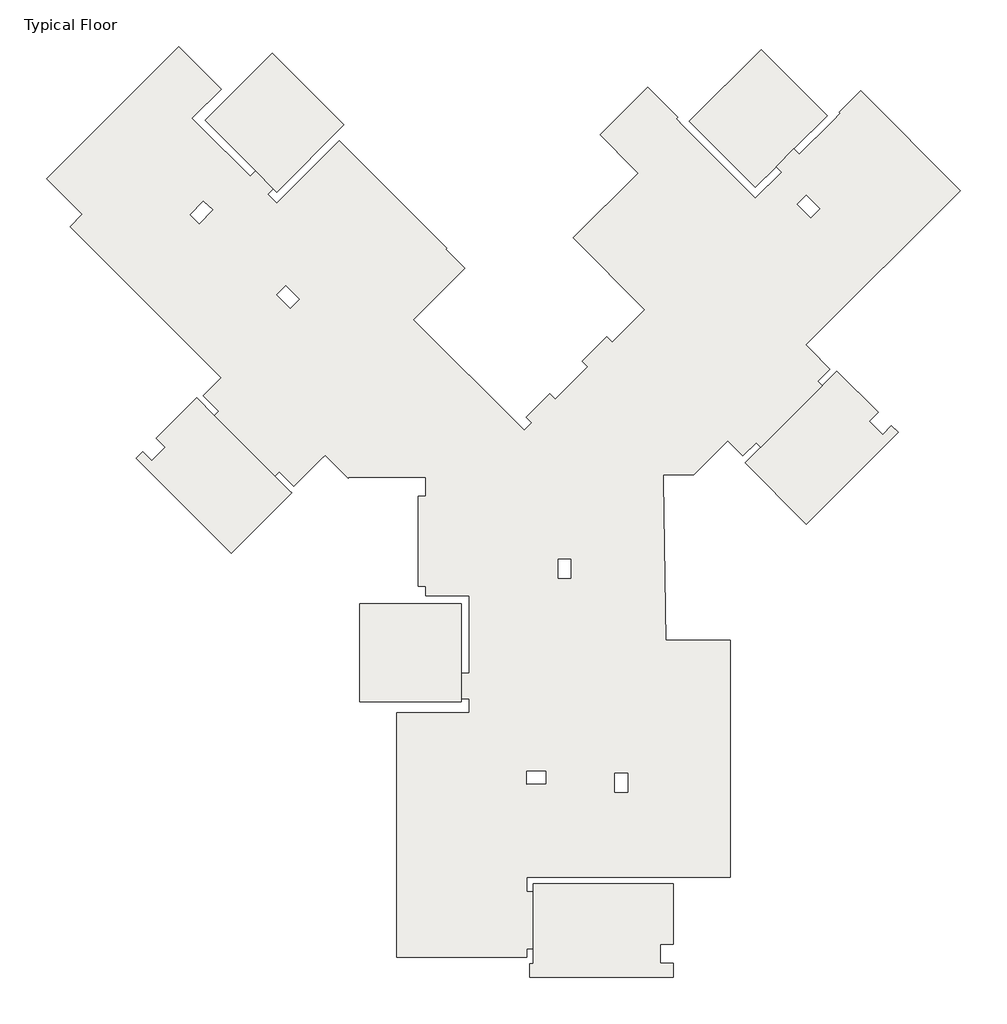
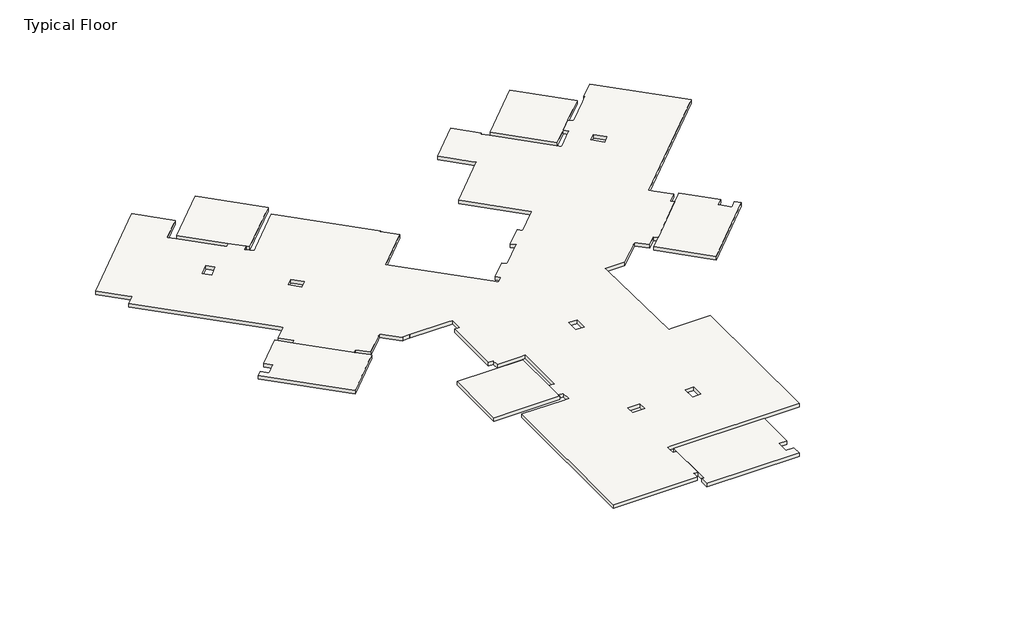
# One storey: 7 slabs.
"""IFC4 building model written with IfcOpenShell, lengths in millimetres."""

from ifc_helpers import new_model, si_unit, origin, place, context, project, spatial, faceted_brep, element, save

model = new_model("IFC4")

# Units and contexts
model_context = context("Model", 3, world=origin())
ifc_project = project(units=[si_unit("LENGTHUNIT", "METRE", prefix="MILLI")], contexts=[model_context])

# Site, building, storey
site = spatial("IfcSite", under=ifc_project)
building = spatial("IfcBuilding", under=site)
storey = spatial("IfcBuildingStorey", under=building, Name="Typical Floor", Elevation=3000.0)

# Slabs
placement = place(None, origin())
element("IfcSlab", 1, ObjectType="18", at=placement, inside=storey, context=model_context, shape_type="Brep", body=[
    faceted_brep([(-7856.4284934, -710.7469277, 2820.0), (-10855.8752998, 2291.0608544, 2820.0), (-10643.7250884, 2503.0442058, 2820.0), (-10362.7349591, 2221.337265, 2820.0), (-9937.9307713, 2645.0605261, 2820.0), (-10219.2939768, 2927.1414948, 2820.0), (-8946.5252944, 4198.9091219, 2820.0), (-8385.3549973, 3637.7388248, 2820.0), (-6476.6083787, 1728.9922062, 2820.0), (-6010.9986053, 1263.3824328, 2820.0), (-5945.8975357, 1198.2813632, 2820.0), (-10855.8752998, 2291.0608544, 3000.0), (-7856.4284934, -710.7469277, 3000.0), (-5945.8975357, 1198.2813632, 3000.0), (-6010.9986053, 1263.3824328, 3000.0), (-6476.6083787, 1728.9922062, 3000.0), (-8385.3549973, 3637.7388248, 3000.0), (-8946.5252944, 4198.9091219, 3000.0), (-10219.2939768, 2927.1414948, 3000.0), (-9937.9307713, 2645.0605261, 3000.0), (-10362.7349591, 2221.337265, 3000.0), (-10643.7250884, 2503.0442058, 3000.0)], [[[0, 1, 2, 3, 4, 5, 6, 7, 8, 9, 10]], [[11, 12, 13, 14, 15, 16, 17, 18, 19, 20, 21]], [[1, 0, 12, 11]], [[1, 11, 21, 2]], [[17, 6, 5, 18]], [[6, 17, 16, 15, 14, 13, 10, 9, 8, 7]], [[0, 10, 13, 12]], [[3, 20, 19, 4]], [[20, 3, 2, 21]], [[4, 19, 18, 5]]]),
])
element("IfcSlab", 2, ObjectType="18", at=placement, inside=storey, context=model_context, shape_type="Brep", body=[
    faceted_brep([(1689.535885, -11158.0646121, 2820.0), (6112.9804297, -11158.0646121, 2820.0), (6112.9804297, -13069.1556852, 2820.0), (5712.9804297, -13069.1556852, 2820.0), (5712.9804297, -13669.1556852, 2820.0), (6112.9804297, -13669.1556852, 2820.0), (6112.9804297, -14118.5695716, 2820.0), (1589.2653711, -14118.5695716, 2820.0), (1589.2653711, -13687.1899503, 2820.0), (1689.535885, -13687.1899503, 2820.0), (1689.535885, -13208.1998691, 2820.0), (1689.535885, -11409.1015824, 2820.0), (6112.9804297, -11158.0646121, 3000.0), (1689.535885, -11158.0646121, 3000.0), (1689.535885, -11409.1015824, 3000.0), (1689.535885, -13208.1998691, 3000.0), (1689.535885, -13687.1899503, 3000.0), (1589.2653711, -13687.1899503, 3000.0), (1589.2653711, -14118.5695716, 3000.0), (6112.9804297, -14118.5695716, 3000.0), (6112.9804297, -13669.1556852, 3000.0), (5712.9804297, -13669.1556852, 3000.0), (5712.9804297, -13069.1556852, 3000.0), (6112.9804297, -13069.1556852, 3000.0)], [[[0, 1, 2, 3, 4, 5, 6, 7, 8, 9, 10, 11]], [[12, 13, 14, 15, 16, 17, 18, 19, 20, 21, 22, 23]], [[1, 0, 13, 12]], [[1, 12, 23, 2]], [[19, 6, 5, 20]], [[7, 6, 19, 18]], [[8, 7, 18, 17]], [[9, 8, 17, 16]], [[9, 16, 15, 14, 13, 0, 11, 10]], [[4, 21, 20, 5]], [[21, 4, 3, 22]], [[22, 3, 2, 23]]]),
])
element("IfcSlab", 3, ObjectType="18", at=placement, inside=storey, context=model_context, shape_type="Brep", body=[
    faceted_brep([(13230.1629629, 3112.966169, 2820.0), (10331.02516, 213.8283661, 2820.0), (8393.4317005, 2151.4218256, 2820.0), (8888.8145144, 2646.8046394, 2820.0), (10826.9573797, 4584.9475048, 2820.0), (11210.8737714, 4968.8638964, 2820.0), (11292.5695034, 5050.5596284, 2820.0), (12593.7668598, 3749.362272, 2820.0), (12310.9241473, 3466.5195596, 2820.0), (12735.188216, 3042.2554908, 2820.0), (13018.0309285, 3325.0982033, 2820.0), (10331.02516, 213.8283661, 3000.0), (13230.1629629, 3112.966169, 3000.0), (13018.0309285, 3325.0982033, 3000.0), (12735.188216, 3042.2554908, 3000.0), (12310.9241473, 3466.5195596, 3000.0), (12593.7668598, 3749.362272, 3000.0), (11292.5695034, 5050.5596284, 3000.0), (11210.8737714, 4968.8638964, 3000.0), (10826.9573797, 4584.9475048, 3000.0), (8888.8145144, 2646.8046394, 3000.0), (8393.4317005, 2151.4218256, 3000.0)], [[[0, 1, 2, 3, 4, 5, 6, 7, 8, 9, 10]], [[11, 12, 13, 14, 15, 16, 17, 18, 19, 20, 21]], [[1, 0, 12, 11]], [[2, 1, 11, 21]], [[2, 21, 20, 19, 18, 17, 6, 5, 4, 3]], [[6, 17, 16, 7]], [[12, 0, 10, 13]], [[9, 14, 13, 10]], [[14, 9, 8, 15]], [[15, 8, 7, 16]]]),
])
element("IfcSlab", 4, ObjectType="18", at=placement, inside=storey, context=model_context, shape_type="Brep", body=[
    faceted_brep([(-4287.1177238, 12828.2129875, 2820.0), (-6408.5705171, 10706.7601941, 2820.0), (-6515.2924693, 10813.4821463, 2820.0), (-7080.4863376, 11378.6760146, 2820.0), (-8671.4119489, 12969.6016259, 2820.0), (-6549.9591555, 15091.0544192, 2820.0), (-6408.5705171, 10706.7601941, 3000.0), (-4287.1177238, 12828.2129875, 3000.0), (-6549.9591555, 15091.0544192, 3000.0), (-8671.4119489, 12969.6016259, 3000.0), (-7080.4863376, 11378.6760146, 3000.0), (-6515.2924693, 10813.4821463, 3000.0)], [[[0, 1, 2, 3, 4, 5]], [[6, 7, 8, 9, 10, 11]], [[1, 0, 7, 6]], [[1, 6, 11, 10, 9, 4, 3, 2]], [[5, 4, 9, 8]], [[0, 5, 8, 7]]]),
])
element("IfcSlab", 5, ObjectType="18", at=placement, inside=storey, context=model_context, shape_type="Brep", body=[
    faceted_brep([(8717.8496812, 10862.5762446, 2820.0), (6632.1047328, 12948.3211931, 2820.0), (8894.9461646, 15211.1626248, 2820.0), (10980.691113, 13125.4176764, 2820.0), (9934.0396226, 12078.766186, 2820.0), (9369.5671248, 11514.2936882, 2820.0), (6632.1047328, 12948.3211931, 3000.0), (8717.8496812, 10862.5762446, 3000.0), (9369.5671248, 11514.2936882, 3000.0), (9934.0396226, 12078.766186, 3000.0), (10980.691113, 13125.4176764, 3000.0), (8894.9461646, 15211.1626248, 3000.0)], [[[0, 1, 2, 3, 4, 5]], [[6, 7, 8, 9, 10, 11]], [[7, 0, 5, 4, 3, 10, 9, 8]], [[1, 0, 7, 6]], [[2, 1, 6, 11]], [[3, 2, 11, 10]]]),
])
element("IfcSlab", 6, ObjectType="18", at=placement, inside=storey, context=model_context, shape_type="Brep", body=[
    faceted_brep([(-576.6949536, -2309.417182, 2820.0), (-576.6949536, -4509.9131243, 2820.0), (-576.6949536, -5309.9131243, 2820.0), (-576.6949536, -5409.3270107, 2820.0), (-3786.2531141, -5409.3270107, 2820.0), (-3786.2531141, -2309.417182, 2820.0), (-576.6949536, -2309.417182, 3000.0), (-3786.2531141, -2309.417182, 3000.0), (-3786.2531141, -2409.417182, 3000.0), (-3786.2531141, -5409.3270107, 3000.0), (-576.6949536, -5409.3270107, 3000.0), (-576.6949536, -5309.9131243, 3000.0), (-576.6949536, -4509.9131243, 3000.0)], [[[0, 1, 2, 3, 4, 5]], [[6, 7, 8, 9, 10, 11, 12]], [[3, 2, 1, 0, 6, 12, 11, 10]], [[4, 3, 10, 9]], [[5, 4, 9, 8, 7]], [[0, 5, 7, 6]]]),
])
element("IfcSlab", 7, ObjectType="18", at=placement, inside=storey, context=model_context, shape_type="Brep", body=[
    faceted_brep([(-8173.4037002, 13962.5846214, 2820.0), (-9095.6760176, 13040.312304, 2820.0), (-8848.1886442, 12792.8249306, 2820.0), (-7257.2630329, 11201.8993193, 2820.0), (-7080.4863376, 11378.6760146, 2820.0), (-6515.2924693, 10813.4821463, 2820.0), (-6692.0691646, 10636.705451, 2820.0), (-6408.5705171, 10353.2068036, 2820.0), (-6231.7938218, 10529.9834989, 2820.0), (-4429.582499, 12332.1948217, 2820.0), (-1033.4026062, 8936.0149288, 2820.0), (-1068.6984287, 8900.7191063, 2820.0), (-468.8867571, 8300.9074348, 2820.0), (-2095.1940493, 6674.6001426, 2820.0), (-1918.417354, 6497.8234473, 2820.0), (1231.0458064, 3348.3602869, 2820.0), (1407.8225017, 3171.5835916, 2820.0), (1655.2707813, 3419.0318712, 2820.0), (1478.494086, 3595.8085665, 2820.0), (2220.7844377, 4338.0989181, 2820.0), (2397.561133, 4161.3222229, 2820.0), (3424.432188, 5188.1932779, 2820.0), (3247.6554927, 5364.9699732, 2820.0), (4022.4075216, 6139.722002, 2820.0), (4199.1842169, 5962.9453067, 2820.0), (5050.3606325, 6814.1217223, 2820.0), (5227.1373278, 6990.8984176, 2820.0), (2962.7877192, 9255.2480262, 2820.0), (5013.5473558, 11306.0076628, 2820.0), (4872.1259995, 11447.429019, 2820.0), (3807.7763909, 12511.7786276, 2820.0), (5320.554821, 14024.5570577, 2820.0), (6266.9603358, 13078.1515429, 2820.0), (6207.8406641, 13019.0318712, 2820.0), (6455.3280375, 12771.5444978, 2820.0), (8541.0729859, 10685.7995493, 2820.0), (8717.8496812, 10509.0228541, 2820.0), (9546.3438201, 11337.5169929, 2820.0), (9369.5671248, 11514.2936882, 2820.0), (9934.0396226, 12078.766186, 2820.0), (10110.8163179, 11901.9894907, 2820.0), (11157.4678083, 12948.6409811, 2820.0), (11404.9551817, 13196.1283545, 2820.0), (11369.6407399, 13231.4427963, 2820.0), (12039.7613133, 13901.5633697, 2820.0), (15186.314453, 10755.0102301, 2820.0), (10305.5209453, 5874.2167224, 2820.0), (10446.9423016, 5732.7953662, 2820.0), (11069.4524151, 5110.2852526, 2820.0), (10685.5360235, 4726.368861, 2820.0), (10826.9573797, 4584.9475048, 2820.0), (8888.8145144, 2646.8046394, 2820.0), (8747.3931582, 2788.2259957, 2820.0), (8323.1290895, 2363.961927, 2820.0), (7842.9320868, 2844.1589296, 2820.0), (7701.5107306, 2702.7375734, 2820.0), (6767.6697714, 1768.8966142, 2820.0), (5805.6765523, 1768.8966142, 2820.0), (5808.4890075, 1568.8966142, 2820.0), (5879.1909347, -3458.8761541, 2820.0), (6079.2107085, -3458.8761541, 2820.0), (7926.5061285, -3458.8761541, 2820.0), (7926.5061285, -10958.0646121, 2820.0), (1689.535885, -10958.0646121, 2820.0), (1489.535885, -10958.0646121, 2820.0), (1489.535885, -11409.1015824, 2820.0), (1689.535885, -11409.1015824, 2820.0), (1689.535885, -13208.1998691, 2820.0), (1489.535885, -13208.1998691, 2820.0), (1489.535885, -13487.1899503, 2820.0), (-2615.4235379, -13487.1899503, 2820.0), (-2615.4235379, -5759.3270107, 2820.0), (-576.6949536, -5759.3270107, 2820.0), (-326.6949536, -5759.3270107, 2820.0), (-326.6949536, -5309.9131243, 2820.0), (-576.6949536, -5309.9131243, 2820.0), (-576.6949536, -4509.9131243, 2820.0), (-326.6949536, -4509.9131243, 2820.0), (-326.6949536, -2059.417182, 2820.0), (-576.6949536, -2059.417182, 2820.0), (-1697.2991014, -2059.417182, 2820.0), (-1697.2991014, -1759.417182, 2820.0), (-1947.2991014, -1759.417182, 2820.0), (-1947.2991014, 1090.0868757, 2820.0), (-1697.2991014, 1090.0868757, 2820.0), (-1697.2991014, 1690.0868757, 2820.0), (-3801.5371537, 1690.0868757, 2820.0), (-3801.5371537, 1690.2672183, 2820.0), (-4151.5371537, 1690.2672183, 2820.0), (-4151.5371537, 1666.662681, 2820.0), (-4879.6277554, 2394.7532827, 2820.0), (-5021.0491116, 2253.3319265, 2820.0), (-5869.5772491, 1404.803789, 2820.0), (-6335.1870225, 1870.4135624, 2820.0), (-6476.6083787, 1728.9922062, 2820.0), (-8385.3549973, 3637.7388248, 2820.0), (-8243.933641, 3779.160181, 2820.0), (-8738.7611577, 4273.9876976, 2820.0), (-8172.2562086, 4840.4926467, 2820.0), (-8313.6775649, 4981.9140029, 2820.0), (-12945.5654963, 9613.8019343, 2820.0), (-12556.7794585, 10002.5879721, 2820.0), (-12698.2008147, 10144.0093284, 2820.0), (-13688.6426542, 11134.4511678, 2820.0), (-9516.9564504, 15306.1373716, 2820.0), (4677.0922421, -8261.9946197, 2820.0), (4677.0922421, -7661.9946197, 2820.0), (4277.0922421, -7661.9946197, 2820.0), (4277.0922421, -8261.9946197, 2820.0), (2484.8469761, -897.4694814, 2820.0), (2484.8469761, -1497.4694814, 2820.0), (2884.8469761, -1497.4694814, 2820.0), (2884.8469761, -897.4694814, 2820.0), (-5702.252807, 7320.6604284, 2820.0), (-6125.9760682, 7745.4646162, 2820.0), (-6409.17886, 7462.9824421, 2820.0), (-5985.4555989, 7038.1782543, 2820.0), (2084.6127194, -7598.6919819, 2820.0), (1484.675203, -7607.3508739, 2820.0), (1490.4477976, -8007.3092182, 2820.0), (2090.385314, -7998.6503262, 2820.0), (10744.1797083, 10180.0778586, 2820.0), (10319.9156396, 10604.3419273, 2820.0), (10037.0729271, 10321.4992148, 2820.0), (10461.3369958, 9897.2351461, 2820.0), (-8856.8048079, 9710.3988417, 2820.0), (-8440.7447422, 10142.7112538, 2820.0), (-8728.9530169, 10420.084631, 2820.0), (-9145.0130827, 9987.7722189, 2820.0), (-9095.6760176, 13040.312304, 3000.0), (-8173.4037002, 13962.5846214, 3000.0), (-9516.9564504, 15306.1373716, 3000.0), (-13688.6426542, 11134.4511678, 3000.0), (-12698.2008147, 10144.0093284, 3000.0), (-12556.7794585, 10002.5879721, 3000.0), (-12945.5654963, 9613.8019343, 3000.0), (-8313.6775649, 4981.9140029, 3000.0), (-8172.2562086, 4840.4926467, 3000.0), (-8738.7611577, 4273.9876976, 3000.0), (-8243.933641, 3779.160181, 3000.0), (-8385.3549973, 3637.7388248, 3000.0), (-6476.6083787, 1728.9922062, 3000.0), (-6335.1870225, 1870.4135624, 3000.0), (-5869.5772491, 1404.803789, 3000.0), (-5021.0491116, 2253.3319265, 3000.0), (-4879.6277554, 2394.7532827, 3000.0), (-4151.5371537, 1666.662681, 3000.0), (-4151.5371537, 1690.2672183, 3000.0), (-3801.5371537, 1690.2672183, 3000.0), (-3801.5371537, 1690.0868757, 3000.0), (-1947.2991014, 1690.0868757, 3000.0), (-1697.2991014, 1690.0868757, 3000.0), (-1697.2991014, 1090.0868757, 3000.0), (-1947.2991014, 1090.0868757, 3000.0), (-1947.2991014, -1759.417182, 3000.0), (-1697.2991014, -1759.417182, 3000.0), (-1697.2991014, -2059.417182, 3000.0), (-576.6949536, -2059.417182, 3000.0), (-326.6949536, -2059.417182, 3000.0), (-326.6949536, -4509.9131243, 3000.0), (-576.6949536, -4509.9131243, 3000.0), (-576.6949536, -5309.9131243, 3000.0), (-326.6949536, -5309.9131243, 3000.0), (-326.6949536, -5759.3270107, 3000.0), (-576.6949536, -5759.3270107, 3000.0), (-2615.4235379, -5759.3270107, 3000.0), (-2615.4235379, -13487.1899503, 3000.0), (1489.535885, -13487.1899503, 3000.0), (1489.535885, -13208.1998691, 3000.0), (1689.535885, -13208.1998691, 3000.0), (1689.535885, -11409.1015824, 3000.0), (1489.535885, -11409.1015824, 3000.0), (1489.535885, -10958.0646121, 3000.0), (1689.535885, -10958.0646121, 3000.0), (7926.5061285, -10958.0646121, 3000.0), (7926.5061285, -3458.8761541, 3000.0), (6079.2107085, -3458.8761541, 3000.0), (5879.1909347, -3458.8761541, 3000.0), (5808.4890075, 1568.8966142, 3000.0), (5805.6765523, 1768.8966142, 3000.0), (6767.6697714, 1768.8966142, 3000.0), (7701.5107306, 2702.7375734, 3000.0), (7842.9320868, 2844.1589296, 3000.0), (8323.1290895, 2363.961927, 3000.0), (8747.3931582, 2788.2259957, 3000.0), (8888.8145144, 2646.8046394, 3000.0), (10826.9573797, 4584.9475048, 3000.0), (10685.5360235, 4726.368861, 3000.0), (11069.4524151, 5110.2852526, 3000.0), (10446.9423016, 5732.7953662, 3000.0), (10305.5209453, 5874.2167224, 3000.0), (15186.314453, 10755.0102301, 3000.0), (12039.7613133, 13901.5633697, 3000.0), (11369.6407399, 13231.4427963, 3000.0), (11404.9551817, 13196.1283545, 3000.0), (11157.4678083, 12948.6409811, 3000.0), (10110.8163179, 11901.9894907, 3000.0), (9934.0396226, 12078.766186, 3000.0), (9369.5671248, 11514.2936882, 3000.0), (9546.3438201, 11337.5169929, 3000.0), (8717.8496812, 10509.0228541, 3000.0), (8541.0729859, 10685.7995493, 3000.0), (6455.3280375, 12771.5444978, 3000.0), (6207.8406641, 13019.0318712, 3000.0), (6266.9603358, 13078.1515429, 3000.0), (5320.554821, 14024.5570577, 3000.0), (3807.7763909, 12511.7786276, 3000.0), (4872.1259995, 11447.429019, 3000.0), (5013.5473558, 11306.0076628, 3000.0), (2962.7877192, 9255.2480262, 3000.0), (5227.1373278, 6990.8984176, 3000.0), (5050.3606325, 6814.1217223, 3000.0), (4199.1842169, 5962.9453067, 3000.0), (4022.4075216, 6139.722002, 3000.0), (3247.6554927, 5364.9699732, 3000.0), (3424.432188, 5188.1932779, 3000.0), (2397.561133, 4161.3222229, 3000.0), (2220.7844377, 4338.0989181, 3000.0), (1478.494086, 3595.8085665, 3000.0), (1655.2707813, 3419.0318712, 3000.0), (1407.8225017, 3171.5835916, 3000.0), (1231.0458064, 3348.3602869, 3000.0), (-1918.417354, 6497.8234473, 3000.0), (-2095.1940493, 6674.6001426, 3000.0), (-468.8867571, 8300.9074348, 3000.0), (-1068.6984287, 8900.7191063, 3000.0), (-1033.4026062, 8936.0149288, 3000.0), (-4429.582499, 12332.1948217, 3000.0), (-6231.7938218, 10529.9834989, 3000.0), (-6408.5705171, 10353.2068036, 3000.0), (-6692.0691646, 10636.705451, 3000.0), (-6515.2924693, 10813.4821463, 3000.0), (-7080.4863376, 11378.6760146, 3000.0), (-7257.2630329, 11201.8993193, 3000.0), (-8848.1886442, 12792.8249306, 3000.0), (4677.0922421, -7661.9946197, 3000.0), (4677.0922421, -8261.9946197, 3000.0), (4277.0922421, -8261.9946197, 3000.0), (4277.0922421, -7661.9946197, 3000.0), (2484.8469761, -1497.4694814, 3000.0), (2484.8469761, -897.4694814, 3000.0), (2884.8469761, -897.4694814, 3000.0), (2884.8469761, -1497.4694814, 3000.0), (-6125.9760682, 7745.4646162, 3000.0), (-5702.252807, 7320.6604284, 3000.0), (-5985.4555989, 7038.1782543, 3000.0), (-6409.17886, 7462.9824421, 3000.0), (1484.675203, -7607.3508739, 3000.0), (2084.6127194, -7598.6919819, 3000.0), (2090.385314, -7998.6503262, 3000.0), (1490.4477976, -8007.3092182, 3000.0), (10319.9156396, 10604.3419273, 3000.0), (10744.1797083, 10180.0778586, 3000.0), (10461.3369958, 9897.2351461, 3000.0), (10037.0729271, 10321.4992148, 3000.0), (-8440.7447422, 10142.7112538, 3000.0), (-8856.8048079, 9710.3988417, 3000.0), (-9145.0130827, 9987.7722189, 3000.0), (-8728.9530169, 10420.084631, 3000.0)], [[[0, 1, 2, 3, 4, 5, 6, 7, 8, 9, 10, 11, 12, 13, 14, 15, 16, 17, 18, 19, 20, 21, 22, 23, 24, 25, 26, 27, 28, 29, 30, 31, 32, 33, 34, 35, 36, 37, 38, 39, 40, 41, 42, 43, 44, 45, 46, 47, 48, 49, 50, 51, 52, 53, 54, 55, 56, 57, 58, 59, 60, 61, 62, 63, 64, 65, 66, 67, 68, 69, 70, 71, 72, 73, 74, 75, 76, 77, 78, 79, 80, 81, 82, 83, 84, 85, 86, 87, 88, 89, 90, 91, 92, 93, 94, 95, 96, 97, 98, 99, 100, 101, 102, 103, 104], [105, 106, 107, 108], [109, 110, 111, 112], [113, 114, 115, 116], [117, 118, 119, 120], [121, 122, 123, 124], [125, 126, 127, 128]], [[129, 130, 131, 132, 133, 134, 135, 136, 137, 138, 139, 140, 141, 142, 143, 144, 145, 146, 147, 148, 149, 150, 151, 152, 153, 154, 155, 156, 157, 158, 159, 160, 161, 162, 163, 164, 165, 166, 167, 168, 169, 170, 171, 172, 173, 174, 175, 176, 177, 178, 179, 180, 181, 182, 183, 184, 185, 186, 187, 188, 189, 190, 191, 192, 193, 194, 195, 196, 197, 198, 199, 200, 201, 202, 203, 204, 205, 206, 207, 208, 209, 210, 211, 212, 213, 214, 215, 216, 217, 218, 219, 220, 221, 222, 223, 224, 225, 226, 227, 228, 229, 230, 231, 232, 233, 234], [235, 236, 237, 238], [239, 240, 241, 242], [243, 244, 245, 246], [247, 248, 249, 250], [251, 252, 253, 254], [255, 256, 257, 258]], [[1, 0, 130, 129]], [[1, 129, 234, 233, 3, 2]], [[4, 3, 233, 232]], [[5, 4, 232, 231]], [[6, 5, 231, 230]], [[7, 6, 230, 229]], [[7, 229, 228, 227, 9, 8]], [[10, 9, 227, 226]], [[11, 10, 226, 225]], [[12, 11, 225, 224]], [[13, 12, 224, 223]], [[13, 223, 222, 221, 220, 16, 15, 14]], [[210, 26, 25, 24, 212, 211]], [[27, 26, 210, 209]], [[28, 27, 209, 208]], [[28, 208, 207, 206, 30, 29]], [[31, 30, 206, 205]], [[32, 31, 205, 204]], [[33, 32, 204, 203]], [[33, 203, 202, 201, 200, 36, 35, 34]], [[37, 36, 200, 199]], [[38, 37, 199, 198]], [[39, 38, 198, 197]], [[40, 39, 197, 196]], [[40, 196, 195, 194, 42, 41]], [[43, 42, 194, 193]], [[44, 43, 193, 192]], [[45, 44, 192, 191]], [[46, 45, 191, 190]], [[46, 190, 189, 188, 48, 47]], [[49, 48, 188, 187]], [[50, 49, 187, 186]], [[51, 50, 186, 185]], [[52, 51, 185, 184]], [[53, 52, 184, 183]], [[54, 53, 183, 182]], [[54, 182, 181, 180, 56, 55]], [[57, 56, 180, 179]], [[57, 179, 178, 177, 59, 58]], [[59, 177, 176, 175, 61, 60]], [[62, 61, 175, 174]], [[62, 174, 173, 172, 64, 63]], [[65, 64, 172, 171]], [[66, 65, 171, 170]], [[67, 66, 170, 169]], [[68, 67, 169, 168]], [[69, 68, 168, 167]], [[70, 69, 167, 166]], [[71, 70, 166, 165]], [[71, 165, 164, 163, 73, 72]], [[74, 73, 163, 162]], [[75, 74, 162, 161]], [[76, 75, 161, 160]], [[77, 76, 160, 159]], [[78, 77, 159, 158]], [[78, 158, 157, 156, 80, 79]], [[146, 89, 88, 147]], [[90, 89, 146, 145]], [[90, 145, 144, 143, 92, 91]], [[93, 92, 143, 142]], [[94, 93, 142, 141]], [[95, 94, 141, 140]], [[96, 95, 140, 139]], [[97, 96, 139, 138]], [[98, 97, 138, 137]], [[98, 137, 136, 135, 100, 99]], [[101, 100, 135, 134]], [[101, 134, 133, 132, 103, 102]], [[104, 103, 132, 131]], [[0, 104, 131, 130]], [[17, 16, 220, 219]], [[18, 17, 219, 218]], [[19, 18, 218, 217]], [[20, 19, 217, 216]], [[21, 20, 216, 215]], [[22, 21, 215, 214]], [[23, 22, 214, 213]], [[24, 23, 213, 212]], [[81, 80, 156, 155]], [[82, 81, 155, 154]], [[83, 82, 154, 153]], [[84, 83, 153, 152]], [[84, 152, 151, 85]], [[105, 236, 235, 106]], [[236, 105, 108, 237]], [[237, 108, 107, 238]], [[238, 107, 106, 235]], [[109, 240, 239, 110]], [[240, 109, 112, 241]], [[241, 112, 111, 242]], [[242, 111, 110, 239]], [[113, 244, 243, 114]], [[244, 113, 116, 245]], [[245, 116, 115, 246]], [[246, 115, 114, 243]], [[117, 248, 247, 118]], [[248, 117, 120, 249]], [[249, 120, 119, 250]], [[250, 119, 118, 247]], [[121, 252, 251, 122]], [[252, 121, 124, 253]], [[253, 124, 123, 254]], [[254, 123, 122, 251]], [[125, 256, 255, 126]], [[256, 125, 128, 257]], [[257, 128, 127, 258]], [[258, 127, 126, 255]], [[148, 87, 86, 149]], [[87, 148, 147, 88]], [[85, 151, 150, 149, 86]]]),
])

save(model, "model.ifc")

# Revit data of these elements
# Type "18"
#   Function = 0
#   Layers, outside or top first: 18 cm "Concrete" (function 1)
# Element 1 (IfcSlab, "18")
#   Mark = "S1"
#   SOFiSTiK_AMG_Comments = ""
#   built-in parameter 1001955 = 2.3558 (stored number, unit not read)
#   Height Offset From Level = 0 cm
#   built-in parameter 1001954 = 1
#   SOFiSTiK_AMG_Scheduled = yes
#   SOFiSTiK_AMG_Adjusted = yes
#   Phase Created = New Construction
#   Materials on its faces: "Concrete"
# Element 2 (IfcSlab, "18")
#   Mark = "S2"
#   SOFiSTiK_AMG_Comments = ""
#   built-in parameter 1001955 = 3.14159 (stored number, unit not read)
#   Height Offset From Level = 0 cm
#   built-in parameter 1001954 = 1
#   SOFiSTiK_AMG_Scheduled = yes
#   SOFiSTiK_AMG_Adjusted = yes
#   Phase Created = New Construction
#   Materials on its faces: "Concrete"
# Element 3 (IfcSlab, "18")
#   Mark = "S3"
#   SOFiSTiK_AMG_Comments = ""
#   built-in parameter 1001955 = -0.785398 (stored number, unit not read)
#   Height Offset From Level = 0 cm
#   built-in parameter 1001954 = 1
#   SOFiSTiK_AMG_Scheduled = yes
#   SOFiSTiK_AMG_Adjusted = yes
#   Phase Created = New Construction
#   Materials on its faces: "Concrete"
# Element 4 (IfcSlab, "18")
#   Mark = "S4"
#   SOFiSTiK_AMG_Comments = ""
#   built-in parameter 1001955 = -0.785398 (stored number, unit not read)
#   Height Offset From Level = 0 cm
#   built-in parameter 1001954 = 1
#   SOFiSTiK_AMG_Scheduled = yes
#   SOFiSTiK_AMG_Adjusted = yes
#   Phase Created = New Construction
#   Materials on its faces: "Concrete"
# Element 5 (IfcSlab, "18")
#   Mark = "S5"
#   SOFiSTiK_AMG_Comments = ""
#   built-in parameter 1001955 = -0.785398 (stored number, unit not read)
#   Height Offset From Level = 0 cm
#   built-in parameter 1001954 = 1
#   SOFiSTiK_AMG_Scheduled = yes
#   SOFiSTiK_AMG_Adjusted = yes
#   Phase Created = New Construction
#   Materials on its faces: "Concrete"
# Element 6 (IfcSlab, "18")
#   Mark = "S6"
#   SOFiSTiK_AMG_Comments = ""
#   Height Offset From Level = 0 cm
#   built-in parameter 1001954 = 1
#   SOFiSTiK_AMG_Scheduled = yes
#   SOFiSTiK_AMG_Adjusted = yes
#   Phase Created = New Construction
#   Materials on its faces: "Concrete"
# Element 7 (IfcSlab, "18")
#   Mark = "S7"
#   SOFiSTiK_AMG_Comments = ""
#   built-in parameter 1001955 = -0.785398 (stored number, unit not read)
#   Height Offset From Level = 0 cm
#   built-in parameter 1001954 = 1
#   SOFiSTiK_AMG_Scheduled = yes
#   SOFiSTiK_AMG_Adjusted = yes
#   Phase Created = New Construction
#   Materials on its faces: "Concrete"
# Materials
#   "Concrete": class "Concrete", colour RGB 192 192 192, transparency 0, Keynote = "01000", Description = "Cast-in-place concrete", Cost = 0
